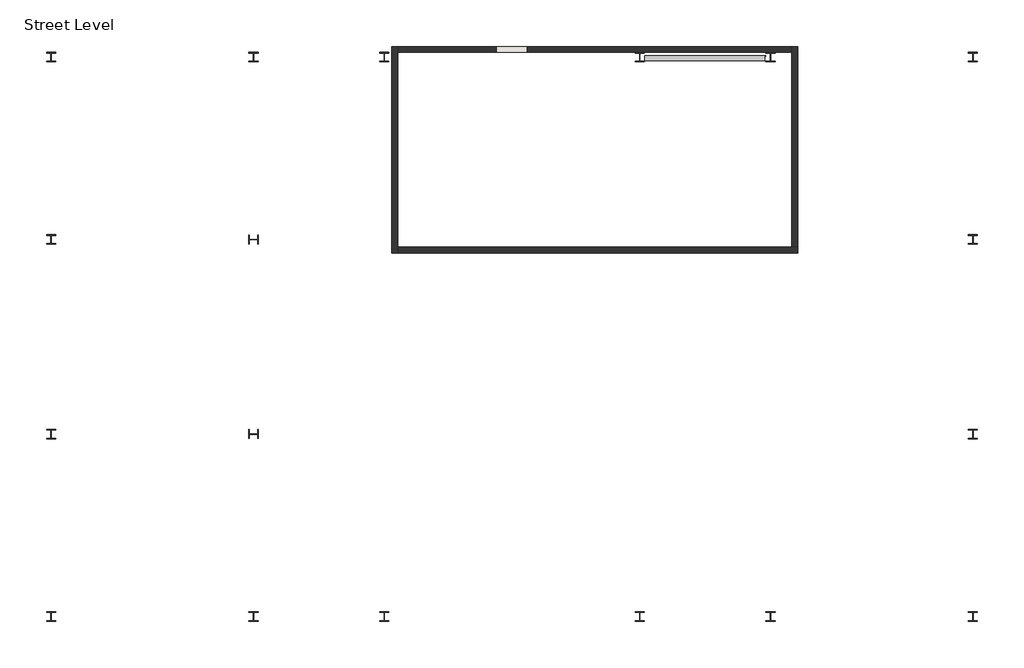
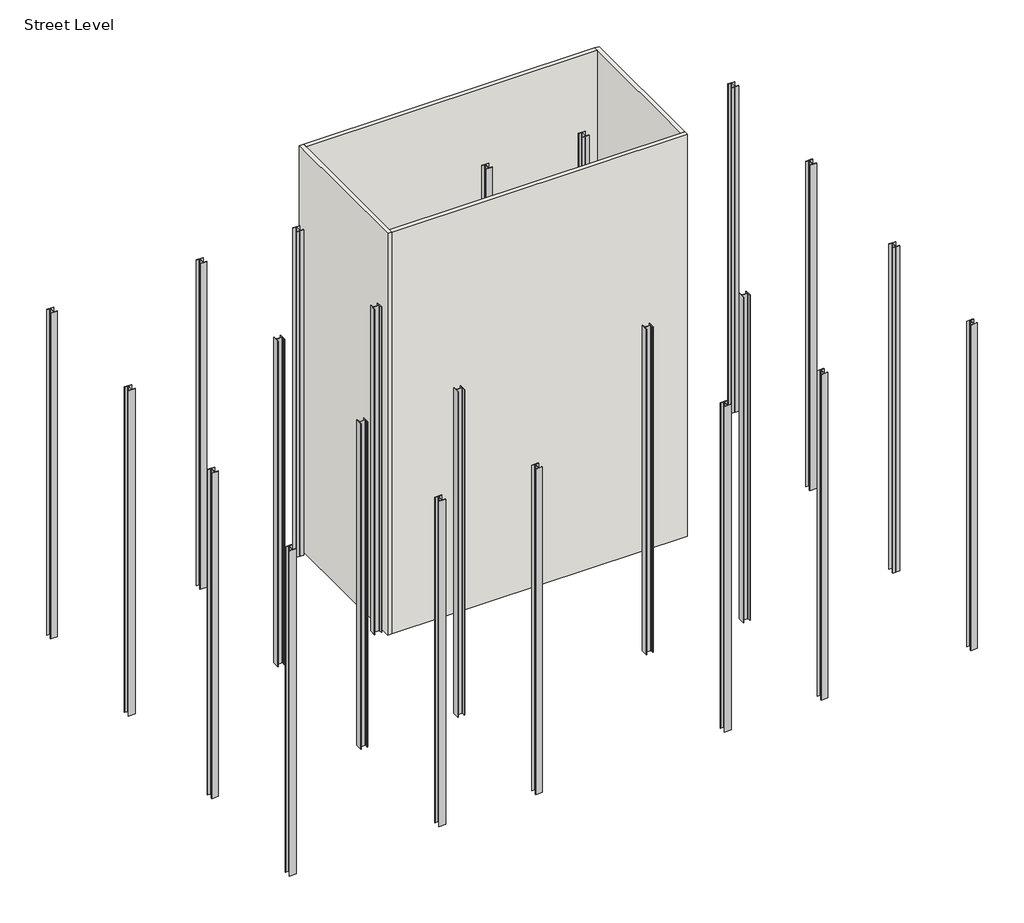
# One storey: 24 columns, 4 walls, 1 member.
"""IFC4 building model written with IfcOpenShell, lengths in millimetres."""

import ifcopenshell
import ifcopenshell.guid

model = None  # the IFC model being written
_history = None  # IfcOwnerHistory: only IFC2X3 demands one
_inside = {}  # id of a spatial element -> (the spatial element, [elements in it])
_under = {}  # id of a project, library or spatial element -> (it, [spatial elements below it])
_declared = {}  # id of a project -> (the project, [libraries it declares])
_typed = {}  # id of a type object -> (the type object, [elements of that type])
_made_of = {}  # id of a material, layer set ... -> (it, [elements and type objects made of it])


def new_model(schema):
    """Start an empty IFC model of exactly this schema.

    Asked for "IFC4X3", IfcOpenShell would pick the latest addendum, in which some entities
    have other attributes; the version numbers below select the first issue.
    IFC2X3 requires an IfcOwnerHistory on every rooted entity: one is made here for all.
    """
    global model, _history
    if schema == "IFC4X3":
        model = ifcopenshell.file(schema_version=(4, 3, 0, 0))
    else:
        model = ifcopenshell.file(schema=schema)
    _inside.clear()
    _under.clear()
    _declared.clear()
    _typed.clear()
    _made_of.clear()
    _history = None
    if model.schema == "IFC2X3":
        org = make("IfcOrganization", Name="unknown")
        user = make(
            "IfcPersonAndOrganization",
            ThePerson=make("IfcPerson", FamilyName="unknown"),
            TheOrganization=org,
        )
        app = make(
            "IfcApplication",
            ApplicationDeveloper=org,
            Version="unknown",
            ApplicationFullName="unknown",
            ApplicationIdentifier="unknown",
        )
        _history = make(
            "IfcOwnerHistory",
            OwningUser=user,
            OwningApplication=app,
            ChangeAction="ADDED",
            CreationDate=0,
        )
    return model


def make(cls, **values):
    """One entity of the class cls with the attributes given. An attribute that is None is left unset."""
    return model.create_entity(
        cls, **{name: value for name, value in values.items() if value is not None}
    )


def rooted(cls, **values):
    """An entity with a GlobalId (a new one), such as an element, a storey or a relation."""
    return make(cls, GlobalId=ifcopenshell.guid.new(), OwnerHistory=_history, **values)


def si_unit(unit_type, name, prefix=None):
    """IfcSIUnit, for example si_unit("LENGTHUNIT", "METRE", prefix="MILLI")."""
    return make("IfcSIUnit", UnitType=unit_type, Prefix=prefix, Name=name)


def assignment(units):
    """IfcUnitAssignment: the units of a project."""
    return None if units is None else make("IfcUnitAssignment", Units=units)


def point(xyz):
    """IfcCartesianPoint."""
    return None if xyz is None else make("IfcCartesianPoint", Coordinates=xyz)


def direction(xyz):
    """IfcDirection."""
    return None if xyz is None else make("IfcDirection", DirectionRatios=xyz)


def frame(location, z_axis=None, x_axis=None):
    """IfcAxis2Placement3D, a coordinate frame: its origin and axes. An axis left out is left unset."""
    return make(
        "IfcAxis2Placement3D",
        Location=point(location),
        Axis=direction(z_axis),
        RefDirection=direction(x_axis),
    )


def frame_2d(location, x_axis=None):
    """IfcAxis2Placement2D, a coordinate frame in the plane: its origin and x axis."""
    return make(
        "IfcAxis2Placement2D", Location=point(location), RefDirection=direction(x_axis)
    )


def origin():
    """The frame at (0, 0, 0) with its axes left unset."""
    return frame((0.0, 0.0, 0.0))


def place(relative_to, where):
    """IfcLocalPlacement: puts the frame where relative to a parent placement (None: the world)."""
    return make(
        "IfcLocalPlacement", PlacementRelTo=relative_to, RelativePlacement=where
    )


def context(
    kind, dimensions, precision=None, world=None, true_north=None, identifier=None
):
    """IfcGeometricRepresentationContext, for example the 3D "Model" context."""
    return make(
        "IfcGeometricRepresentationContext",
        ContextIdentifier=identifier,
        ContextType=kind,
        CoordinateSpaceDimension=dimensions,
        Precision=precision,
        WorldCoordinateSystem=world,
        TrueNorth=true_north,
    )


def project(units=None, contexts=None):
    """IfcProject with its units and contexts."""
    return rooted(
        "IfcProject",
        Name="project",
        RepresentationContexts=contexts,
        UnitsInContext=assignment(units),
    )


def spatial(cls, under=None, at=None, **own):
    """A site, building, storey or space (cls), placed at a placement, below another one or the project."""
    s = rooted(cls, ObjectPlacement=at, **own)
    if under is not None:
        _under.setdefault(under.id(), (under, []))[1].append(s)
    return s


def polyline(points):
    """IfcPolyline through the points."""
    return make("IfcPolyline", Points=[point(p) for p in points])


def circle_curve(where, radius):
    """IfcCircle in the frame where."""
    return make("IfcCircle", Position=where, Radius=radius)


def trimmed(basis, trim1, trim2, sense, master):
    """IfcTrimmedCurve: the piece of a basis curve between two trims."""
    return make(
        "IfcTrimmedCurve",
        BasisCurve=basis,
        Trim1=trim1,
        Trim2=trim2,
        SenseAgreement=sense,
        MasterRepresentation=master,
    )


def segment(curve, same_sense, transition):
    """IfcCompositeCurveSegment."""
    return make(
        "IfcCompositeCurveSegment",
        Transition=transition,
        SameSense=same_sense,
        ParentCurve=curve,
    )


def composite_curve(segments, self_intersect=None):
    """IfcCompositeCurve: segments joined end to end."""
    return make("IfcCompositeCurve", Segments=segments, SelfIntersect=self_intersect)


def outline(outer, holes=None, kind="AREA"):
    """IfcArbitraryClosedProfileDef: a profile drawn as a closed curve; with holes, ...WithVoids."""
    if holes is None:
        return make("IfcArbitraryClosedProfileDef", ProfileType=kind, OuterCurve=outer)
    return make(
        "IfcArbitraryProfileDefWithVoids",
        ProfileType=kind,
        OuterCurve=outer,
        InnerCurves=holes,
    )


def extrude(swept, where, along, depth):
    """IfcExtrudedAreaSolid: the profile swept, set in the frame where, extruded along a direction by depth."""
    return make(
        "IfcExtrudedAreaSolid",
        SweptArea=swept,
        Position=where,
        ExtrudedDirection=direction(along),
        Depth=depth,
    )


def faces_of(points, faces, orient=None, outer=None):
    """IfcFace entities. A face is a list of loops; a loop is a list of indices into points, from 0.

    orient and outer hold one flag for each loop. By default every Orientation is true, the
    first loop of a face is its IfcFaceOuterBound and the others are IfcFaceBound.
    """
    made = []
    for i, loops in enumerate(faces):
        bounds = []
        for j, loop in enumerate(loops):
            is_outer = j == 0 if outer is None else outer[i][j]
            bounds.append(
                make(
                    "IfcFaceOuterBound" if is_outer else "IfcFaceBound",
                    Bound=make("IfcPolyLoop", Polygon=[points[k] for k in loop]),
                    Orientation=True if orient is None else orient[i][j],
                )
            )
        made.append(make("IfcFace", Bounds=bounds))
    return made


def faceted_brep(points, faces, orient=None, outer=None, voids=None):
    """IfcFacetedBrep: a solid bounded by flat faces; with voids (closed shells), ...WithVoids."""
    shared = [point(p) for p in points]
    hull = make("IfcClosedShell", CfsFaces=faces_of(shared, faces, orient, outer))
    if voids is None:
        return make("IfcFacetedBrep", Outer=hull)
    return make(
        "IfcFacetedBrepWithVoids",
        Outer=hull,
        Voids=[
            make(cls, CfsFaces=faces_of(shared, fs, o, b)) for cls, fs, o, b in voids
        ],
    )


def shape(context_of_items, identifier, shape_type, items):
    """IfcShapeRepresentation: the items that make up one representation, for example the "Body"."""
    return make(
        "IfcShapeRepresentation",
        ContextOfItems=context_of_items,
        RepresentationIdentifier=identifier,
        RepresentationType=shape_type,
        Items=items,
    )


def source(mapping_origin, context_of_items, identifier, shape_type, items):
    """IfcRepresentationMap: a shape defined once, which mapped items show again and again."""
    return make(
        "IfcRepresentationMap",
        MappingOrigin=mapping_origin,
        MappedRepresentation=shape(context_of_items, identifier, shape_type, items),
    )


def transform(
    local_origin,
    x_axis=None,
    y_axis=None,
    z_axis=None,
    scale=None,
    scale2=None,
    scale3=None,
    uniform=True,
):
    """IfcCartesianTransformationOperator3D, or its non-uniform kind. x_axis, y_axis, z_axis: its Axis1, 2, 3."""
    if uniform:
        return make(
            "IfcCartesianTransformationOperator3D",
            Axis1=direction(x_axis),
            Axis2=direction(y_axis),
            LocalOrigin=point(local_origin),
            Scale=scale,
            Axis3=direction(z_axis),
        )
    return make(
        "IfcCartesianTransformationOperator3DnonUniform",
        Axis1=direction(x_axis),
        Axis2=direction(y_axis),
        LocalOrigin=point(local_origin),
        Scale=scale,
        Axis3=direction(z_axis),
        Scale2=scale2,
        Scale3=scale3,
    )


def mapped(mapping_source, mapping_target):
    """IfcMappedItem: shows the shape of a source again, moved by a transform."""
    return make(
        "IfcMappedItem", MappingSource=mapping_source, MappingTarget=mapping_target
    )


def made_of(thing, what):
    """Note that an element or type object is made of a material, layer set ...; save() writes the relation."""
    if what is not None:
        _made_of.setdefault(what.id(), (what, []))[1].append(thing)
    return thing


def element(
    cls,
    number,
    at=None,
    inside=None,
    cuts=None,
    type_object=None,
    material=None,
    context=None,
    identifier="Body",
    shape_type=None,
    held_by="IfcProductDefinitionShape",
    body=None,
    shapes=None,
    **own,
):
    """One element of the class cls, such as IfcWall. Its Tag is "e" and its number.

    at: its placement. inside: the storey or other place that contains it. cuts: it is an
    opening in that element (IfcRelVoidsElement). A single representation is given by context,
    identifier, shape_type and body (its items); several are given by shapes. held_by: the class
    of the entity that holds the representations. save() writes the other relations.
    """
    e = rooted(cls, Tag="e%d" % number, ObjectPlacement=at, **own)
    if body is not None:
        shapes = [shape(context, identifier, shape_type, body)]
    if shapes is not None:
        e.Representation = make(held_by, Representations=shapes)
    if inside is not None:
        _inside.setdefault(inside.id(), (inside, []))[1].append(e)
    if cuts is not None:
        rooted(
            "IfcRelVoidsElement", RelatingBuildingElement=cuts, RelatedOpeningElement=e
        )
    if type_object is not None:
        _typed.setdefault(type_object.id(), (type_object, []))[1].append(e)
    return made_of(e, material)


def aggregate(whole, parts):
    """IfcRelAggregates: a whole, such as a stair, and the parts it consists of."""
    return rooted("IfcRelAggregates", RelatingObject=whole, RelatedObjects=parts)


def save(model, path):
    """Write the relations noted so far, then the file.

    IfcRelAggregates (storeys below a building ...), IfcRelContainedInSpatialStructure (elements
    in a storey), IfcRelDefinesByType, IfcRelAssociatesMaterial and IfcRelDeclares: one each for
    every whole, place, type object, material and project.
    """
    for whole, parts in _under.values():
        aggregate(whole, parts)
    for where, things in _inside.values():
        rooted(
            "IfcRelContainedInSpatialStructure",
            RelatedElements=things,
            RelatingStructure=where,
        )
    for kind, things in _typed.values():
        rooted("IfcRelDefinesByType", RelatedObjects=things, RelatingType=kind)
    for what, things in _made_of.values():
        rooted("IfcRelAssociatesMaterial", RelatedObjects=things, RelatingMaterial=what)
    for by, libraries in _declared.values():
        rooted("IfcRelDeclares", RelatingContext=by, RelatedDefinitions=libraries)
    model.write(path)


def w_wide_flange_column_w12x87_da20b1fb(model_context):
    return source(origin(), model_context, "Body", "SweptSolid", [
        extrude(outline(composite_curve([segment(polyline([(153.9875, 159.146875), (153.9875, 138.6085937), (28.8726562, 138.6085937)]), True, "CONTINUOUS"), segment(trimmed(circle_curve(frame_2d((28.8726562, 116.284375)), 22.3242188), [point((28.8726562, 138.6085937))], [point((6.5484375, 116.284375))], True, "CARTESIAN"), True, "CONTINUOUS"), segment(polyline([(6.5484375, 116.284375), (6.5484375, -116.284375)]), True, "CONTINUOUS"), segment(trimmed(circle_curve(frame_2d((28.8726562, -116.284375)), 22.3242188), [point((6.5484375, -116.284375))], [point((28.8726562, -138.6085937))], True, "CARTESIAN"), True, "CONTINUOUS"), segment(polyline([(28.8726562, -138.6085937), (153.9875, -138.6085937), (153.9875, -159.146875), (-153.9875, -159.146875), (-153.9875, -138.6085937), (-28.8726563, -138.6085937)]), True, "CONTINUOUS"), segment(trimmed(circle_curve(frame_2d((-28.8726563, -116.284375)), 22.3242188), [point((-28.8726563, -138.6085937))], [point((-6.5484375, -116.284375))], True, "CARTESIAN"), True, "CONTINUOUS"), segment(polyline([(-6.5484375, -116.284375), (-6.5484375, 116.284375)]), True, "CONTINUOUS"), segment(trimmed(circle_curve(frame_2d((-28.8726563, 116.284375)), 22.3242188), [point((-6.5484375, 116.284375))], [point((-28.8726563, 138.6085937))], True, "CARTESIAN"), True, "CONTINUOUS"), segment(polyline([(-28.8726563, 138.6085937), (-153.9875, 138.6085937), (-153.9875, 159.146875), (153.9875, 159.146875)]), True, "CONTINUOUS")], self_intersect=False)), frame((0.0, 0.0, -914.4), z_axis=(0.0, 0.0, 1.0), x_axis=(1.0, 0.0, 0.0)), (0.0, 0.0, 1.0), 15544.8),
    ])


def l_angle2_l6x6x3_8_670392f0(model_context):
    return source(origin(), model_context, "Body", "SweptSolid", [
        extrude(outline(composite_curve([segment(polyline([(41.148, 41.148), (41.148, -111.252)]), True, "CONTINUOUS"), segment(trimmed(circle_curve(frame_2d((41.148, -101.727)), 9.525), [point((41.148, -111.252))], [point((31.623, -101.727))], False, "CARTESIAN"), True, "CONTINUOUS"), segment(polyline([(31.623, -101.727), (31.623, 22.098)]), True, "CONTINUOUS"), segment(trimmed(circle_curve(frame_2d((22.098, 22.098)), 9.525), [point((31.623, 22.098))], [point((22.098, 31.623))], True, "CARTESIAN"), True, "CONTINUOUS"), segment(polyline([(22.098, 31.623), (-101.727, 31.623)]), True, "CONTINUOUS"), segment(trimmed(circle_curve(frame_2d((-101.727, 41.148)), 9.525), [point((-101.727, 31.623))], [point((-111.252, 41.148))], False, "CARTESIAN"), True, "CONTINUOUS"), segment(polyline([(-111.252, 41.148), (41.148, 41.148)]), True, "CONTINUOUS")], self_intersect=False)), frame((-2053.0970548, 0.0, 0.0), z_axis=(1.0, 0.0, 0.0), x_axis=(0.0, 1.0, 0.0)), (0.0, 0.0, 1.0), 4091.5211794),
    ])


model = new_model("IFC4")

# Units and contexts
model_context = context("Model", 3, world=origin())
ifc_project = project(units=[si_unit("LENGTHUNIT", "METRE", prefix="MILLI")], contexts=[model_context])

# Site, building, storey
site = spatial("IfcSite", under=ifc_project)
building = spatial("IfcBuilding", under=site)
storey = spatial("IfcBuildingStorey", under=building, Name="Street Level", Elevation=-914.4)

# Columns
placement = place(None, origin())
w_wide_flange_column_w12x87_shape = w_wide_flange_column_w12x87_da20b1fb(model_context)
element("IfcColumn", 1, ObjectType="W-Wide Flange-Column : W12X87", at=placement, inside=storey, context=model_context, shape_type="MappedRepresentation", body=[
    mapped(w_wide_flange_column_w12x87_shape, transform((-9801.8122732, -3408.4984696, 0.0), x_axis=(0.0, -1.0, 0.0), y_axis=(1.0, 0.0, 0.0), z_axis=(0.0, 0.0, 1.0))),
])
element("IfcColumn", 2, ObjectType="W-Wide Flange-Column : W12X87", at=placement, inside=storey, context=model_context, shape_type="MappedRepresentation", body=[
    mapped(w_wide_flange_column_w12x87_shape, transform((-5433.0122732, -3408.4984696, 0.0), x_axis=(0.0, -1.0, 0.0), y_axis=(1.0, 0.0, 0.0), z_axis=(0.0, 0.0, 1.0))),
])
element("IfcColumn", 3, ObjectType="W-Wide Flange-Column : W12X87", at=placement, inside=storey, context=model_context, shape_type="MappedRepresentation", body=[
    mapped(w_wide_flange_column_w12x87_shape, transform((3101.3877268, -3408.4984696, 0.0), x_axis=(0.0, -1.0, 0.0), y_axis=(1.0, 0.0, 0.0), z_axis=(0.0, 0.0, 1.0))),
])
element("IfcColumn", 4, ObjectType="W-Wide Flange-Column : W12X87", at=placement, inside=storey, context=model_context, shape_type="MappedRepresentation", body=[
    mapped(w_wide_flange_column_w12x87_shape, transform((7470.1877268, -3408.4984696, 0.0), x_axis=(0.0, -1.0, 0.0), y_axis=(1.0, 0.0, 0.0), z_axis=(0.0, 0.0, 1.0))),
])
element("IfcColumn", 5, ObjectType="W-Wide Flange-Column : W12X87", at=placement, inside=storey, context=model_context, shape_type="MappedRepresentation", body=[
    mapped(w_wide_flange_column_w12x87_shape, transform((-9801.8122732, 3093.9015304, 0.0), x_axis=(0.0, -1.0, 0.0), y_axis=(1.0, 0.0, 0.0), z_axis=(0.0, 0.0, 1.0))),
])
element("IfcColumn", 6, ObjectType="W-Wide Flange-Column : W12X87", at=placement, inside=storey, context=model_context, shape_type="MappedRepresentation", body=[
    mapped(w_wide_flange_column_w12x87_shape, transform((-5433.0122732, 3093.9015304, 0.0), x_axis=(0.0, -1.0, 0.0), y_axis=(1.0, 0.0, 0.0), z_axis=(0.0, 0.0, 1.0))),
])
element("IfcColumn", 7, ObjectType="W-Wide Flange-Column : W12X87", at=placement, inside=storey, context=model_context, shape_type="MappedRepresentation", body=[
    mapped(w_wide_flange_column_w12x87_shape, transform((3101.3877268, 3093.9015304, 0.0), x_axis=(0.0, -1.0, 0.0), y_axis=(1.0, 0.0, 0.0), z_axis=(0.0, 0.0, 1.0))),
])
element("IfcColumn", 8, ObjectType="W-Wide Flange-Column : W12X87", at=placement, inside=storey, context=model_context, shape_type="MappedRepresentation", body=[
    mapped(w_wide_flange_column_w12x87_shape, transform((7470.1877268, 3093.9015304, 0.0), x_axis=(0.0, -1.0, 0.0), y_axis=(1.0, 0.0, 0.0), z_axis=(0.0, 0.0, 1.0))),
])
element("IfcColumn", 9, ObjectType="W-Wide Flange-Column : W12X87", at=placement, inside=storey, context=model_context, shape_type="MappedRepresentation", body=[
    mapped(w_wide_flange_column_w12x87_shape, transform((-16558.2122732, 9189.9015304, 0.0), x_axis=(1.0, 0.0, 0.0), y_axis=(0.0, 1.0, 0.0), z_axis=(0.0, 0.0, 1.0))),
])
element("IfcColumn", 10, ObjectType="W-Wide Flange-Column : W12X87", at=placement, inside=storey, context=model_context, shape_type="MappedRepresentation", body=[
    mapped(w_wide_flange_column_w12x87_shape, transform((-16558.2122732, 3093.9015304, 0.0), x_axis=(1.0, 0.0, 0.0), y_axis=(0.0, 1.0, 0.0), z_axis=(0.0, 0.0, 1.0))),
])
element("IfcColumn", 11, ObjectType="W-Wide Flange-Column : W12X87", at=placement, inside=storey, context=model_context, shape_type="MappedRepresentation", body=[
    mapped(w_wide_flange_column_w12x87_shape, transform((-9801.8122732, 9189.9015304, 0.0), x_axis=(1.0, 0.0, 0.0), y_axis=(0.0, 1.0, 0.0), z_axis=(0.0, 0.0, 1.0))),
])
element("IfcColumn", 12, ObjectType="W-Wide Flange-Column : W12X87", at=placement, inside=storey, context=model_context, shape_type="MappedRepresentation", body=[
    mapped(w_wide_flange_column_w12x87_shape, transform((-5433.0122732, 9189.9015304, 0.0), x_axis=(1.0, 0.0, 0.0), y_axis=(0.0, 1.0, 0.0), z_axis=(0.0, 0.0, 1.0))),
])
element("IfcColumn", 13, ObjectType="W-Wide Flange-Column : W12X87", at=placement, inside=storey, context=model_context, shape_type="MappedRepresentation", body=[
    mapped(w_wide_flange_column_w12x87_shape, transform((3101.3877268, 9189.9015304, 0.0), x_axis=(1.0, 0.0, 0.0), y_axis=(0.0, 1.0, 0.0), z_axis=(0.0, 0.0, 1.0))),
])
element("IfcColumn", 14, ObjectType="W-Wide Flange-Column : W12X87", at=placement, inside=storey, context=model_context, shape_type="MappedRepresentation", body=[
    mapped(w_wide_flange_column_w12x87_shape, transform((7470.1877268, 9189.9015304, 0.0), x_axis=(1.0, 0.0, 0.0), y_axis=(0.0, 1.0, 0.0), z_axis=(0.0, 0.0, 1.0))),
])
element("IfcColumn", 15, ObjectType="W-Wide Flange-Column : W12X87", at=placement, inside=storey, context=model_context, shape_type="MappedRepresentation", body=[
    mapped(w_wide_flange_column_w12x87_shape, transform((14226.5877268, 9189.9015304, 0.0), x_axis=(1.0, 0.0, 0.0), y_axis=(0.0, 1.0, 0.0), z_axis=(0.0, 0.0, 1.0))),
])
element("IfcColumn", 16, ObjectType="W-Wide Flange-Column : W12X87", at=placement, inside=storey, context=model_context, shape_type="MappedRepresentation", body=[
    mapped(w_wide_flange_column_w12x87_shape, transform((14226.5877268, 3093.9015304, 0.0), x_axis=(1.0, 0.0, 0.0), y_axis=(0.0, 1.0, 0.0), z_axis=(0.0, 0.0, 1.0))),
])
element("IfcColumn", 17, ObjectType="W-Wide Flange-Column : W12X87", at=placement, inside=storey, context=model_context, shape_type="MappedRepresentation", body=[
    mapped(w_wide_flange_column_w12x87_shape, transform((14226.5877268, -3408.4984696, 0.0), x_axis=(1.0, 0.0, 0.0), y_axis=(0.0, 1.0, 0.0), z_axis=(0.0, 0.0, 1.0))),
])
element("IfcColumn", 18, ObjectType="W-Wide Flange-Column : W12X87", at=placement, inside=storey, context=model_context, shape_type="MappedRepresentation", body=[
    mapped(w_wide_flange_column_w12x87_shape, transform((14226.5877268, -9504.4984696, 0.0), x_axis=(1.0, 0.0, 0.0), y_axis=(0.0, 1.0, 0.0), z_axis=(0.0, 0.0, 1.0))),
])
element("IfcColumn", 19, ObjectType="W-Wide Flange-Column : W12X87", at=placement, inside=storey, context=model_context, shape_type="MappedRepresentation", body=[
    mapped(w_wide_flange_column_w12x87_shape, transform((7470.1877268, -9504.4984696, 0.0), x_axis=(1.0, 0.0, 0.0), y_axis=(0.0, 1.0, 0.0), z_axis=(0.0, 0.0, 1.0))),
])
element("IfcColumn", 20, ObjectType="W-Wide Flange-Column : W12X87", at=placement, inside=storey, context=model_context, shape_type="MappedRepresentation", body=[
    mapped(w_wide_flange_column_w12x87_shape, transform((3101.3877268, -9504.4984696, 0.0), x_axis=(1.0, 0.0, 0.0), y_axis=(0.0, 1.0, 0.0), z_axis=(0.0, 0.0, 1.0))),
])
element("IfcColumn", 21, ObjectType="W-Wide Flange-Column : W12X87", at=placement, inside=storey, context=model_context, shape_type="MappedRepresentation", body=[
    mapped(w_wide_flange_column_w12x87_shape, transform((-5433.0122732, -9504.4984696, 0.0), x_axis=(1.0, 0.0, 0.0), y_axis=(0.0, 1.0, 0.0), z_axis=(0.0, 0.0, 1.0))),
])
element("IfcColumn", 22, ObjectType="W-Wide Flange-Column : W12X87", at=placement, inside=storey, context=model_context, shape_type="MappedRepresentation", body=[
    mapped(w_wide_flange_column_w12x87_shape, transform((-9801.8122732, -9504.4984696, 0.0), x_axis=(1.0, 0.0, 0.0), y_axis=(0.0, 1.0, 0.0), z_axis=(0.0, 0.0, 1.0))),
])
element("IfcColumn", 23, ObjectType="W-Wide Flange-Column : W12X87", at=placement, inside=storey, context=model_context, shape_type="MappedRepresentation", body=[
    mapped(w_wide_flange_column_w12x87_shape, transform((-16558.2122732, -9504.4984696, 0.0), x_axis=(1.0, 0.0, 0.0), y_axis=(0.0, 1.0, 0.0), z_axis=(0.0, 0.0, 1.0))),
])
element("IfcColumn", 24, ObjectType="W-Wide Flange-Column : W12X87", at=placement, inside=storey, context=model_context, shape_type="MappedRepresentation", body=[
    mapped(w_wide_flange_column_w12x87_shape, transform((-16558.2122732, -3408.4984696, 0.0), x_axis=(1.0, 0.0, 0.0), y_axis=(0.0, 1.0, 0.0), z_axis=(0.0, 0.0, 1.0))),
])

# Member
l_angle2_l6x6x3_8_shape = l_angle2_l6x6x3_8_670392f0(model_context)
element("IfcMember", 25, ObjectType="L-Angle2 : L6X6X3/8", at=placement, inside=storey, context=model_context, shape_type="MappedRepresentation", body=[
    mapped(l_angle2_l6x6x3_8_shape, transform((5285.7877268, 9189.9015304, -457.2), x_axis=(0.9787906252528689, 0.0, 0.20486315412269337), y_axis=(0.0, 1.0000000000000002, 0.0), z_axis=(-0.20486315412269337, 0.0, 0.9787906252528689))),
])

# Walls
element("IfcWall", 26, ObjectType="Generic - 8\" Masonry", at=placement, inside=storey, context=model_context, shape_type="Brep", body=[
    faceted_brep([(-5174.2497732, 9545.5015304, -914.4), (-5174.2497732, 2641.4640304, -914.4), (-5174.2497732, 2641.4640304, 18288.0), (-5174.2497732, 9545.5015304, 18288.0), (-4980.5747732, 9545.5015304, -914.4), (-4980.5747732, 9545.5015304, 18288.0), (-4980.5747732, 9351.8265304, 18288.0), (-4980.5747732, 2835.1390304, 18288.0), (-4980.5747732, 2641.4640304, 18288.0), (-4980.5747732, 2641.4640304, -914.4), (-4980.5747732, 2835.1390304, -914.4), (-4980.5747732, 9351.8265304, -914.4)], [[[0, 1, 2, 3]], [[4, 5, 6, 7, 8, 9, 10, 11]], [[1, 0, 4, 11, 10, 9]], [[3, 2, 8, 7, 6, 5]], [[2, 1, 9, 8]], [[0, 3, 5, 4]]]),
])
element("IfcWall", 27, ObjectType="Generic - 8\" Masonry", at=placement, inside=storey, context=model_context, shape_type="Brep", body=[
    faceted_brep([(8379.8252268, 2835.1390304, -914.4), (8186.1502268, 2835.1390304, -914.4), (-4980.5747732, 2835.1390304, -914.4), (-4980.5747732, 2835.1390304, 18288.0), (8186.1502268, 2835.1390304, 18288.0), (8379.8252268, 2835.1390304, 18288.0), (8379.8252268, 2641.4640304, -914.4), (8379.8252268, 2641.4640304, 18288.0), (-4980.5747732, 2641.4640304, 18288.0), (-4980.5747732, 2641.4640304, -914.4)], [[[0, 1, 2, 3, 4, 5]], [[6, 7, 8, 9]], [[2, 1, 0, 6, 9]], [[5, 4, 3, 8, 7]], [[0, 5, 7, 6]], [[3, 2, 9, 8]]]),
])
element("IfcWall", 28, ObjectType="Generic - 8\" Masonry", at=placement, inside=storey, context=model_context, shape_type="Brep", body=[
    faceted_brep([(8186.1502268, 9545.5015304, -914.4), (8186.1502268, 9351.8265304, -914.4), (8186.1502268, 2835.1390304, -914.4), (8186.1502268, 2835.1390304, 18288.0), (8186.1502268, 9351.8265304, 18288.0), (8186.1502268, 9545.5015304, 18288.0), (8379.8252268, 9545.5015304, -914.4), (8379.8252268, 9545.5015304, 18288.0), (8379.8252268, 2835.1390304, 18288.0), (8379.8252268, 2835.1390304, -914.4)], [[[0, 1, 2, 3, 4, 5]], [[6, 7, 8, 9]], [[2, 1, 0, 6, 9]], [[5, 4, 3, 8, 7]], [[0, 5, 7, 6]], [[3, 2, 9, 8]]]),
])
element("IfcWall", 29, ObjectType="Generic - 8\" Masonry", at=placement, inside=storey, context=model_context, shape_type="SweptSolid", body=[
    extrude(outline(polyline([(-914.4, -4980.5747732), (-914.4, 8186.1502268), (18288.0, 8186.1502268), (18288.0, -4980.5747732), (-914.4, -4980.5747732)]), holes=[polyline([(2235.2, -1692.8622732), (2235.2, -657.8122732), (0.0, -657.8122732), (0.0, -1692.8622732), (2235.2, -1692.8622732)])]), frame((0.0, 9351.8265304, 0.0), z_axis=(0.0, 1.0, 0.0), x_axis=(0.0, 0.0, 1.0)), (0.0, 0.0, 1.0), 193.675),
])

save(model, "model.ifc")

# Revit data of these elements
# Project information
#   Author = "Paul F. Aubin"
#   Project Issue Date = "8/1/2020"
#   Project Status = "Design Development"
#   Client Name = "Groups and Links"
#   Project Address = "123 State Street, Chicago, IL 60601"
#   Project Name = "07 Commercial-Structure_Complete"
#   Project Number = "2020.01S"
# Grids (mm)
#   "1": line (-22547.601, -9504.498) -> (19277.595, -9504.498)
#   "2": line (-22547.601, -3408.498) -> (19277.595, -3408.498)
#   "3": line (-22547.601, 3093.902) -> (19277.595, 3093.902)
#   "4": line (-22547.601, 9189.902) -> (19277.595, 9189.902)
#   "A": line (-16558.212, 12259.726) -> (-16558.212, -14197.104)
#   "B": line (-9801.812, 12259.726) -> (-9801.812, -14197.104)
#   "C": line (-5433.012, 12259.726) -> (-5433.012, -14197.104)
#   "D": line (3101.388, 12259.726) -> (3101.388, -14197.104)
#   "E": line (7470.188, 12259.726) -> (7470.188, -14197.104)
#   "F": line (14226.588, 12259.726) -> (14226.588, -14197.104)
#   "C.3": line (-2689.812, -15151.11) -> (-2689.812, -5965.346)
#   "C.7": line (358.188, -15151.11) -> (358.188, -5965.346)
# Type "W-Wide Flange-Column : W12X87"
#   Assembly Code = "B10"
#   A = 0.18 SF
#   W = 87
#   bf = 1' - 0 1/8"
#   d = 1' - 0 17/32"
#   k = 0' - 1 11/16"
#   kr = 0' - 0 225/256"
#   tf = 0' - 0 207/256"
#   tw = 0' - 0 33/64"
#   Structural Material [instance default] = Metal - Steel - ASTM A992
# Type "L-Angle2 : L6X6X3/8"
#   Assembly Code = "B10"
#   k = 0' - 0 7/8"
#   W = 14.9
#   Length [instance default] = 5' - 0"
#   b = 0' - 6"
#   d = 0' - 6"
#   t = 0' - 0 3/8"
#   x = 0' - 1.62"
#   y = 0' - 1.62"
#   A = 0.0304167 SF
#   Structural Material [instance default] = Steel ASTM A36
# Type "Generic - 8\" Masonry"
#   Assembly Code = "B2010"
#   Layers, outside or top first: 0' - 7 5/8" "Masonry - Concrete Masonry Units" (function 1)
# Elements 1, 2, 3, 4, 5, 6, 7, 8, 9, 10, 11, 12, 13, 14, 15, 16, 17, 18, 19, 20, 21, 22, 23, 24 (IfcColumn, "W-Wide Flange-Column : W12X87")
#   Structural Material = Metal - Steel - ASTM A992
#   Phase Created = New Construction
#   Materials on its faces: "Metal - Steel - ASTM A992"
# Element 25 (IfcMember, "L-Angle2 : L6X6X3/8")
#   Structural Material = Steel ASTM A36
#   Phase Created = New Construction
#   Materials on its faces: "Steel ASTM A36"
# Elements 26, 27, 28, 29 (IfcWall, "Generic - 8\" Masonry")
#   Top Offset = 12' - 0"
#   Base Offset = 0' - 0"
#   Unconnected Height = 63' - 0"
#   wall height = 63' - 0"
#   Phase Created = New Construction
#   Base Constraint = Street Level
#   Top Constraint = Roof
#   Materials on its faces: "Masonry - Concrete Masonry Units"
# Materials
#   "Metal - Steel - ASTM A992": class "Unassigned", colour RGB 199 199 199, transparency 0, Description = "Steel ASTM A992"
#   "Steel ASTM A36": class "Metal", colour RGB 199 199 199, transparency 0, Description = "Structural steel, ASTM A36 Grade B, mill finish", Cost = 0
#   "Masonry - Concrete Masonry Units": class "Unassigned", colour RGB 227 227 227, transparency 0, Description = "CMU"
